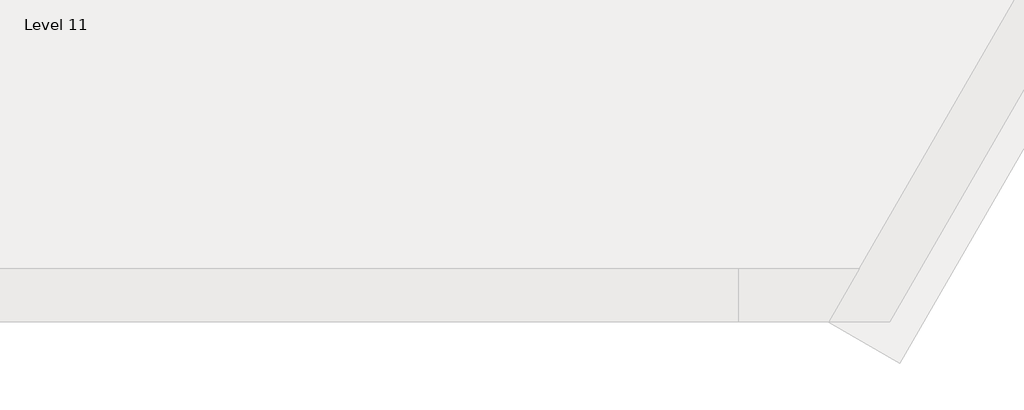
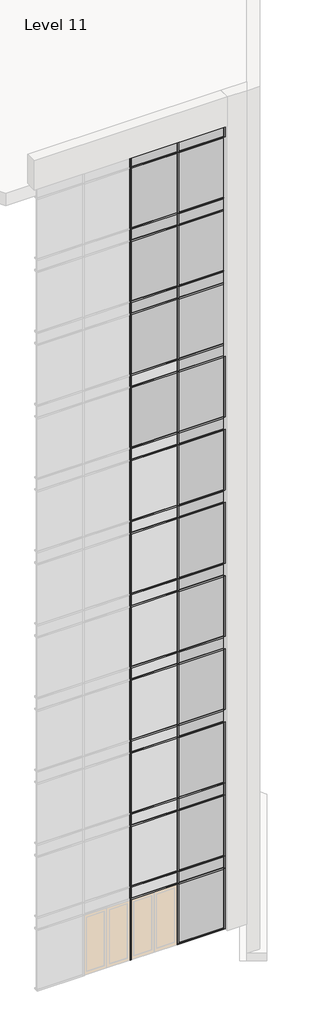
# One storey, part 3 of 6: 100 members, 29 plates.
"""IFC4 building model written with IfcOpenShell, lengths in millimetres."""

import ifcopenshell
import ifcopenshell.guid

model = None  # the IFC model being written
_history = None  # IfcOwnerHistory: only IFC2X3 demands one
_inside = {}  # id of a spatial element -> (the spatial element, [elements in it])
_under = {}  # id of a project, library or spatial element -> (it, [spatial elements below it])
_declared = {}  # id of a project -> (the project, [libraries it declares])
_typed = {}  # id of a type object -> (the type object, [elements of that type])
_made_of = {}  # id of a material, layer set ... -> (it, [elements and type objects made of it])


def new_model(schema):
    """Start an empty IFC model of exactly this schema.

    Asked for "IFC4X3", IfcOpenShell would pick the latest addendum, in which some entities
    have other attributes; the version numbers below select the first issue.
    IFC2X3 requires an IfcOwnerHistory on every rooted entity: one is made here for all.
    """
    global model, _history
    if schema == "IFC4X3":
        model = ifcopenshell.file(schema_version=(4, 3, 0, 0))
    else:
        model = ifcopenshell.file(schema=schema)
    _inside.clear()
    _under.clear()
    _declared.clear()
    _typed.clear()
    _made_of.clear()
    _history = None
    if model.schema == "IFC2X3":
        org = make("IfcOrganization", Name="unknown")
        user = make(
            "IfcPersonAndOrganization",
            ThePerson=make("IfcPerson", FamilyName="unknown"),
            TheOrganization=org,
        )
        app = make(
            "IfcApplication",
            ApplicationDeveloper=org,
            Version="unknown",
            ApplicationFullName="unknown",
            ApplicationIdentifier="unknown",
        )
        _history = make(
            "IfcOwnerHistory",
            OwningUser=user,
            OwningApplication=app,
            ChangeAction="ADDED",
            CreationDate=0,
        )
    return model


def make(cls, **values):
    """One entity of the class cls with the attributes given. An attribute that is None is left unset."""
    return model.create_entity(
        cls, **{name: value for name, value in values.items() if value is not None}
    )


def rooted(cls, **values):
    """An entity with a GlobalId (a new one), such as an element, a storey or a relation."""
    return make(cls, GlobalId=ifcopenshell.guid.new(), OwnerHistory=_history, **values)


def si_unit(unit_type, name, prefix=None):
    """IfcSIUnit, for example si_unit("LENGTHUNIT", "METRE", prefix="MILLI")."""
    return make("IfcSIUnit", UnitType=unit_type, Prefix=prefix, Name=name)


def assignment(units):
    """IfcUnitAssignment: the units of a project."""
    return None if units is None else make("IfcUnitAssignment", Units=units)


def point(xyz):
    """IfcCartesianPoint."""
    return None if xyz is None else make("IfcCartesianPoint", Coordinates=xyz)


def direction(xyz):
    """IfcDirection."""
    return None if xyz is None else make("IfcDirection", DirectionRatios=xyz)


def frame(location, z_axis=None, x_axis=None):
    """IfcAxis2Placement3D, a coordinate frame: its origin and axes. An axis left out is left unset."""
    return make(
        "IfcAxis2Placement3D",
        Location=point(location),
        Axis=direction(z_axis),
        RefDirection=direction(x_axis),
    )


def origin():
    """The frame at (0, 0, 0) with its axes left unset."""
    return frame((0.0, 0.0, 0.0))


def origin_with_axes():
    """The frame at (0, 0, 0) with the z axis (0, 0, 1) and the x axis (1, 0, 0) written out."""
    return frame((0.0, 0.0, 0.0), z_axis=(0.0, 0.0, 1.0), x_axis=(1.0, 0.0, 0.0))


def place(relative_to, where):
    """IfcLocalPlacement: puts the frame where relative to a parent placement (None: the world)."""
    return make(
        "IfcLocalPlacement", PlacementRelTo=relative_to, RelativePlacement=where
    )


def context(
    kind, dimensions, precision=None, world=None, true_north=None, identifier=None
):
    """IfcGeometricRepresentationContext, for example the 3D "Model" context."""
    return make(
        "IfcGeometricRepresentationContext",
        ContextIdentifier=identifier,
        ContextType=kind,
        CoordinateSpaceDimension=dimensions,
        Precision=precision,
        WorldCoordinateSystem=world,
        TrueNorth=true_north,
    )


def project(units=None, contexts=None):
    """IfcProject with its units and contexts."""
    return rooted(
        "IfcProject",
        Name="project",
        RepresentationContexts=contexts,
        UnitsInContext=assignment(units),
    )


def spatial(cls, under=None, at=None, **own):
    """A site, building, storey or space (cls), placed at a placement, below another one or the project."""
    s = rooted(cls, ObjectPlacement=at, **own)
    if under is not None:
        _under.setdefault(under.id(), (under, []))[1].append(s)
    return s


def polyline(points):
    """IfcPolyline through the points."""
    return make("IfcPolyline", Points=[point(p) for p in points])


def outline(outer, holes=None, kind="AREA"):
    """IfcArbitraryClosedProfileDef: a profile drawn as a closed curve; with holes, ...WithVoids."""
    if holes is None:
        return make("IfcArbitraryClosedProfileDef", ProfileType=kind, OuterCurve=outer)
    return make(
        "IfcArbitraryProfileDefWithVoids",
        ProfileType=kind,
        OuterCurve=outer,
        InnerCurves=holes,
    )


def extrude(swept, where, along, depth):
    """IfcExtrudedAreaSolid: the profile swept, set in the frame where, extruded along a direction by depth."""
    return make(
        "IfcExtrudedAreaSolid",
        SweptArea=swept,
        Position=where,
        ExtrudedDirection=direction(along),
        Depth=depth,
    )


def shape(context_of_items, identifier, shape_type, items):
    """IfcShapeRepresentation: the items that make up one representation, for example the "Body"."""
    return make(
        "IfcShapeRepresentation",
        ContextOfItems=context_of_items,
        RepresentationIdentifier=identifier,
        RepresentationType=shape_type,
        Items=items,
    )


def source(mapping_origin, context_of_items, identifier, shape_type, items):
    """IfcRepresentationMap: a shape defined once, which mapped items show again and again."""
    return make(
        "IfcRepresentationMap",
        MappingOrigin=mapping_origin,
        MappedRepresentation=shape(context_of_items, identifier, shape_type, items),
    )


def transform(
    local_origin,
    x_axis=None,
    y_axis=None,
    z_axis=None,
    scale=None,
    scale2=None,
    scale3=None,
    uniform=True,
):
    """IfcCartesianTransformationOperator3D, or its non-uniform kind. x_axis, y_axis, z_axis: its Axis1, 2, 3."""
    if uniform:
        return make(
            "IfcCartesianTransformationOperator3D",
            Axis1=direction(x_axis),
            Axis2=direction(y_axis),
            LocalOrigin=point(local_origin),
            Scale=scale,
            Axis3=direction(z_axis),
        )
    return make(
        "IfcCartesianTransformationOperator3DnonUniform",
        Axis1=direction(x_axis),
        Axis2=direction(y_axis),
        LocalOrigin=point(local_origin),
        Scale=scale,
        Axis3=direction(z_axis),
        Scale2=scale2,
        Scale3=scale3,
    )


def mapped(mapping_source, mapping_target):
    """IfcMappedItem: shows the shape of a source again, moved by a transform."""
    return make(
        "IfcMappedItem", MappingSource=mapping_source, MappingTarget=mapping_target
    )


def made_of(thing, what):
    """Note that an element or type object is made of a material, layer set ...; save() writes the relation."""
    if what is not None:
        _made_of.setdefault(what.id(), (what, []))[1].append(thing)
    return thing


def element(
    cls,
    number,
    at=None,
    inside=None,
    cuts=None,
    type_object=None,
    material=None,
    context=None,
    identifier="Body",
    shape_type=None,
    held_by="IfcProductDefinitionShape",
    body=None,
    shapes=None,
    **own,
):
    """One element of the class cls, such as IfcWall. Its Tag is "e" and its number.

    at: its placement. inside: the storey or other place that contains it. cuts: it is an
    opening in that element (IfcRelVoidsElement). A single representation is given by context,
    identifier, shape_type and body (its items); several are given by shapes. held_by: the class
    of the entity that holds the representations. save() writes the other relations.
    """
    e = rooted(cls, Tag="e%d" % number, ObjectPlacement=at, **own)
    if body is not None:
        shapes = [shape(context, identifier, shape_type, body)]
    if shapes is not None:
        e.Representation = make(held_by, Representations=shapes)
    if inside is not None:
        _inside.setdefault(inside.id(), (inside, []))[1].append(e)
    if cuts is not None:
        rooted(
            "IfcRelVoidsElement", RelatingBuildingElement=cuts, RelatedOpeningElement=e
        )
    if type_object is not None:
        _typed.setdefault(type_object.id(), (type_object, []))[1].append(e)
    return made_of(e, material)


def aggregate(whole, parts):
    """IfcRelAggregates: a whole, such as a stair, and the parts it consists of."""
    return rooted("IfcRelAggregates", RelatingObject=whole, RelatedObjects=parts)


def save(model, path):
    """Write the relations noted so far, then the file.

    IfcRelAggregates (storeys below a building ...), IfcRelContainedInSpatialStructure (elements
    in a storey), IfcRelDefinesByType, IfcRelAssociatesMaterial and IfcRelDeclares: one each for
    every whole, place, type object, material and project.
    """
    for whole, parts in _under.values():
        aggregate(whole, parts)
    for where, things in _inside.values():
        rooted(
            "IfcRelContainedInSpatialStructure",
            RelatedElements=things,
            RelatingStructure=where,
        )
    for kind, things in _typed.values():
        rooted("IfcRelDefinesByType", RelatedObjects=things, RelatingType=kind)
    for what, things in _made_of.values():
        rooted("IfcRelAssociatesMaterial", RelatedObjects=things, RelatingMaterial=what)
    for by, libraries in _declared.values():
        rooted("IfcRelDeclares", RelatingContext=by, RelatedDefinitions=libraries)
    model.write(path)


def rectangular_mullion_50x150mm_86d49a4b(model_context):
    return source(origin(), model_context, "Body", "SweptSolid", [
        extrude(outline(polyline([(0.0, 75.0), (0.0, -75.0), (-50.0, -75.0), (-50.0, 75.0), (0.0, 75.0)])), frame((0.0, 0.0, -1755.0), z_axis=(0.0, 0.0, 1.0), x_axis=(1.0, 0.0, 0.0)), (0.0, 0.0, 1.0), 1755.0),
    ])


def rectangular_mullion_50x150mm_eb9201c3(model_context):
    return source(origin(), model_context, "Body", "SweptSolid", [
        extrude(outline(polyline([(25.0, 75.0), (25.0, -75.0), (-25.0, -75.0), (-25.0, 75.0), (25.0, 75.0)])), frame((0.0, 0.0, -2500.0), z_axis=(0.0, 0.0, 1.0), x_axis=(1.0, 0.0, 0.0)), (0.0, 0.0, 1.0), 2500.0),
    ])


def rectangular_mullion_50x150mm_df7bd136(model_context):
    return source(origin(), model_context, "Body", "SweptSolid", [
        extrude(outline(polyline([(25.0, 75.0), (25.0, -75.0), (-25.0, -75.0), (-25.0, 75.0), (25.0, 75.0)])), frame((0.0, 0.0, -1755.0), z_axis=(0.0, 0.0, 1.0), x_axis=(1.0, 0.0, 0.0)), (0.0, 0.0, 1.0), 1755.0),
    ])


def rectangular_mullion_50x150mm_f5b8645b(model_context):
    return source(origin(), model_context, "Body", "SweptSolid", [
        extrude(outline(polyline([(25.0, 75.0), (25.0, -75.0), (-25.0, -75.0), (-25.0, 75.0), (25.0, 75.0)])), frame((0.0, 0.0, -1780.0), z_axis=(0.0, 0.0, 1.0), x_axis=(1.0, 0.0, 0.0)), (0.0, 0.0, 1.0), 1780.0),
    ])


def rectangular_mullion_50x150mm_ded00a16(model_context):
    return source(origin(), model_context, "Body", "SweptSolid", [
        extrude(outline(polyline([(0.0, 75.0), (0.0, -75.0), (-50.0, -75.0), (-50.0, 75.0), (0.0, 75.0)])), frame((0.0, 0.0, -1780.0), z_axis=(0.0, 0.0, 1.0), x_axis=(1.0, 0.0, 0.0)), (0.0, 0.0, 1.0), 1780.0),
    ])


def rectangular_mullion_50x150mm_22f77a7a(model_context):
    return source(origin(), model_context, "Body", "SweptSolid", [
        extrude(outline(polyline([(25.0, 75.0), (25.0, -75.0), (-25.0, -75.0), (-25.0, 75.0), (25.0, 75.0)])), frame((0.0, 0.0, -500.0), z_axis=(0.0, 0.0, 1.0), x_axis=(1.0, 0.0, 0.0)), (0.0, 0.0, 1.0), 500.0),
    ])


def rectangular_mullion_50x150mm_b3666dbd(model_context):
    return source(origin(), model_context, "Body", "SweptSolid", [
        extrude(outline(polyline([(0.0, 75.0), (0.0, -75.0), (-50.0, -75.0), (-50.0, 75.0), (0.0, 75.0)])), frame((0.0, 0.0, -500.0), z_axis=(0.0, 0.0, 1.0), x_axis=(1.0, 0.0, 0.0)), (0.0, 0.0, 1.0), 500.0),
    ])


def rectangular_mullion_50x150mm_4c3b9bdb(model_context):
    return source(origin(), model_context, "Body", "SweptSolid", [
        extrude(outline(polyline([(0.0, 75.0), (0.0, -75.0), (-50.0, -75.0), (-50.0, 75.0), (0.0, 75.0)])), frame((0.0, 0.0, -2500.0), z_axis=(0.0, 0.0, 1.0), x_axis=(1.0, 0.0, 0.0)), (0.0, 0.0, 1.0), 2500.0),
    ])


def system_panel_glazed_e1ffc32d(model_context):
    return source(origin(), model_context, "Body", "SweptSolid", [
        extrude(outline(polyline([(877.5, 24.5), (-877.5, 24.5), (-877.5, 49.5), (877.5, 49.5), (877.5, 24.5)])), origin_with_axes(), (0.0, 0.0, 1.0), 2425.0),
    ])


def system_panel_glazed_b225d226(model_context):
    return source(origin(), model_context, "Body", "SweptSolid", [
        extrude(outline(polyline([(877.5, 24.5), (-877.5, 24.5), (-877.5, 49.5), (877.5, 49.5), (877.5, 24.5)])), origin_with_axes(), (0.0, 0.0, 1.0), 450.0),
    ])


def system_panel_glazed_87c86ac8(model_context):
    return source(origin(), model_context, "Body", "SweptSolid", [
        extrude(outline(polyline([(890.0, 24.5), (-890.0, 24.5), (-890.0, 49.5), (890.0, 49.5), (890.0, 24.5)])), origin_with_axes(), (0.0, 0.0, 1.0), 450.0),
    ])


def system_panel_glazed_9668c591(model_context):
    return source(origin(), model_context, "Body", "SweptSolid", [
        extrude(outline(polyline([(877.5, 24.5), (-877.5, 24.5), (-877.5, 49.5), (877.5, 49.5), (877.5, 24.5)])), origin_with_axes(), (0.0, 0.0, 1.0), 2450.0),
    ])


def system_panel_glazed_3dade0f0(model_context):
    return source(origin(), model_context, "Body", "SweptSolid", [
        extrude(outline(polyline([(890.0, 24.5), (-890.0, 24.5), (-890.0, 49.5), (890.0, 49.5), (890.0, 24.5)])), origin_with_axes(), (0.0, 0.0, 1.0), 2450.0),
    ])


def system_panel_glazed_44ebf714(model_context):
    return source(origin(), model_context, "Body", "SweptSolid", [
        extrude(outline(polyline([(877.5, 24.5), (-877.5, 24.5), (-877.5, 49.5), (877.5, 49.5), (877.5, 24.5)])), origin_with_axes(), (0.0, 0.0, 1.0), 425.0),
    ])


def system_panel_glazed_68b51738(model_context):
    return source(origin(), model_context, "Body", "SweptSolid", [
        extrude(outline(polyline([(890.0, 24.5), (-890.0, 24.5), (-890.0, 49.5), (890.0, 49.5), (890.0, 24.5)])), origin_with_axes(), (0.0, 0.0, 1.0), 425.0),
    ])


model = new_model("IFC4")

# Units and contexts
model_context = context("Model", 3, world=origin())
ifc_project = project(units=[si_unit("LENGTHUNIT", "METRE", prefix="MILLI")], contexts=[model_context])

# Site, building, storey
site = spatial("IfcSite", under=ifc_project)
building = spatial("IfcBuilding", under=site)
storey = spatial("IfcBuildingStorey", under=building, Name="Level 11", Elevation=33000.0)

# Members
placement = place(None, origin())
rectangular_mullion_50x150mm_shape = rectangular_mullion_50x150mm_86d49a4b(model_context)
element("IfcMember", 1, ObjectType="Rectangular Mullion : 50x150mm", at=placement, inside=storey, context=model_context, shape_type="MappedRepresentation", body=[
    mapped(rectangular_mullion_50x150mm_shape, transform((3638.5639559, -8316.0631989, 0.0), x_axis=(0.0, 0.0, -1.0), y_axis=(0.0, 1.0, 0.0), z_axis=(1.0, 0.0, 0.0))),
])
rectangular_mullion_50x150mm_2_shape = rectangular_mullion_50x150mm_eb9201c3(model_context)
element("IfcMember", 2, ObjectType="Rectangular Mullion : 50x150mm", at=placement, inside=storey, context=model_context, shape_type="MappedRepresentation", body=[
    mapped(rectangular_mullion_50x150mm_2_shape, transform((1858.5639559, -8316.0631989, 0.0), x_axis=(-1.0, 0.0, 0.0), y_axis=(0.0, 1.0, 0.0), z_axis=(0.0, 0.0, -1.0))),
])
element("IfcMember", 3, ObjectType="Rectangular Mullion : 50x150mm", at=placement, inside=storey, context=model_context, shape_type="MappedRepresentation", body=[
    mapped(rectangular_mullion_50x150mm_2_shape, transform((28.5639559, -8316.0631989, 0.0), x_axis=(-1.0, 0.0, 0.0), y_axis=(0.0, 1.0, 0.0), z_axis=(0.0, 0.0, -1.0))),
])
rectangular_mullion_50x150mm_3_shape = rectangular_mullion_50x150mm_df7bd136(model_context)
element("IfcMember", 4, ObjectType="Rectangular Mullion : 50x150mm", at=placement, inside=storey, context=model_context, shape_type="MappedRepresentation", body=[
    mapped(rectangular_mullion_50x150mm_3_shape, transform((1883.5639559, -8316.0631989, 2500.0), x_axis=(0.0, 0.0, 1.0), y_axis=(0.0, 1.0, 0.0), z_axis=(-1.0, 0.0, 0.0))),
])
element("IfcMember", 5, ObjectType="Rectangular Mullion : 50x150mm", at=placement, inside=storey, context=model_context, shape_type="MappedRepresentation", body=[
    mapped(rectangular_mullion_50x150mm_3_shape, transform((1883.5639559, -8316.0631989, 5500.0), x_axis=(0.0, 0.0, 1.0), y_axis=(0.0, 1.0, 0.0), z_axis=(-1.0, 0.0, 0.0))),
])
element("IfcMember", 6, ObjectType="Rectangular Mullion : 50x150mm", at=placement, inside=storey, context=model_context, shape_type="MappedRepresentation", body=[
    mapped(rectangular_mullion_50x150mm_3_shape, transform((1883.5639559, -8316.0631989, 8500.0), x_axis=(0.0, 0.0, 1.0), y_axis=(0.0, 1.0, 0.0), z_axis=(-1.0, 0.0, 0.0))),
])
element("IfcMember", 7, ObjectType="Rectangular Mullion : 50x150mm", at=placement, inside=storey, context=model_context, shape_type="MappedRepresentation", body=[
    mapped(rectangular_mullion_50x150mm_3_shape, transform((1883.5639559, -8316.0631989, 11500.0), x_axis=(0.0, 0.0, 1.0), y_axis=(0.0, 1.0, 0.0), z_axis=(-1.0, 0.0, 0.0))),
])
element("IfcMember", 8, ObjectType="Rectangular Mullion : 50x150mm", at=placement, inside=storey, context=model_context, shape_type="MappedRepresentation", body=[
    mapped(rectangular_mullion_50x150mm_3_shape, transform((1883.5639559, -8316.0631989, 14500.0), x_axis=(0.0, 0.0, 1.0), y_axis=(0.0, 1.0, 0.0), z_axis=(-1.0, 0.0, 0.0))),
])
element("IfcMember", 9, ObjectType="Rectangular Mullion : 50x150mm", at=placement, inside=storey, context=model_context, shape_type="MappedRepresentation", body=[
    mapped(rectangular_mullion_50x150mm_3_shape, transform((1883.5639559, -8316.0631989, 17500.0), x_axis=(0.0, 0.0, 1.0), y_axis=(0.0, 1.0, 0.0), z_axis=(-1.0, 0.0, 0.0))),
])
element("IfcMember", 10, ObjectType="Rectangular Mullion : 50x150mm", at=placement, inside=storey, context=model_context, shape_type="MappedRepresentation", body=[
    mapped(rectangular_mullion_50x150mm_3_shape, transform((1883.5639559, -8316.0631989, 20500.0), x_axis=(0.0, 0.0, 1.0), y_axis=(0.0, 1.0, 0.0), z_axis=(-1.0, 0.0, 0.0))),
])
element("IfcMember", 11, ObjectType="Rectangular Mullion : 50x150mm", at=placement, inside=storey, context=model_context, shape_type="MappedRepresentation", body=[
    mapped(rectangular_mullion_50x150mm_3_shape, transform((1883.5639559, -8316.0631989, 23500.0), x_axis=(0.0, 0.0, 1.0), y_axis=(0.0, 1.0, 0.0), z_axis=(-1.0, 0.0, 0.0))),
])
element("IfcMember", 12, ObjectType="Rectangular Mullion : 50x150mm", at=placement, inside=storey, context=model_context, shape_type="MappedRepresentation", body=[
    mapped(rectangular_mullion_50x150mm_3_shape, transform((1883.5639559, -8316.0631989, 3000.0), x_axis=(0.0, 0.0, 1.0), y_axis=(0.0, 1.0, 0.0), z_axis=(-1.0, 0.0, 0.0))),
])
element("IfcMember", 13, ObjectType="Rectangular Mullion : 50x150mm", at=placement, inside=storey, context=model_context, shape_type="MappedRepresentation", body=[
    mapped(rectangular_mullion_50x150mm_3_shape, transform((1883.5639559, -8316.0631989, 6000.0), x_axis=(0.0, 0.0, 1.0), y_axis=(0.0, 1.0, 0.0), z_axis=(-1.0, 0.0, 0.0))),
])
element("IfcMember", 14, ObjectType="Rectangular Mullion : 50x150mm", at=placement, inside=storey, context=model_context, shape_type="MappedRepresentation", body=[
    mapped(rectangular_mullion_50x150mm_3_shape, transform((1883.5639559, -8316.0631989, 9000.0), x_axis=(0.0, 0.0, 1.0), y_axis=(0.0, 1.0, 0.0), z_axis=(-1.0, 0.0, 0.0))),
])
element("IfcMember", 15, ObjectType="Rectangular Mullion : 50x150mm", at=placement, inside=storey, context=model_context, shape_type="MappedRepresentation", body=[
    mapped(rectangular_mullion_50x150mm_3_shape, transform((1883.5639559, -8316.0631989, 12000.0), x_axis=(0.0, 0.0, 1.0), y_axis=(0.0, 1.0, 0.0), z_axis=(-1.0, 0.0, 0.0))),
])
element("IfcMember", 16, ObjectType="Rectangular Mullion : 50x150mm", at=placement, inside=storey, context=model_context, shape_type="MappedRepresentation", body=[
    mapped(rectangular_mullion_50x150mm_3_shape, transform((1883.5639559, -8316.0631989, 15000.0), x_axis=(0.0, 0.0, 1.0), y_axis=(0.0, 1.0, 0.0), z_axis=(-1.0, 0.0, 0.0))),
])
element("IfcMember", 17, ObjectType="Rectangular Mullion : 50x150mm", at=placement, inside=storey, context=model_context, shape_type="MappedRepresentation", body=[
    mapped(rectangular_mullion_50x150mm_3_shape, transform((1883.5639559, -8316.0631989, 18000.0), x_axis=(0.0, 0.0, 1.0), y_axis=(0.0, 1.0, 0.0), z_axis=(-1.0, 0.0, 0.0))),
])
element("IfcMember", 18, ObjectType="Rectangular Mullion : 50x150mm", at=placement, inside=storey, context=model_context, shape_type="MappedRepresentation", body=[
    mapped(rectangular_mullion_50x150mm_3_shape, transform((1883.5639559, -8316.0631989, 21000.0), x_axis=(0.0, 0.0, 1.0), y_axis=(0.0, 1.0, 0.0), z_axis=(-1.0, 0.0, 0.0))),
])
element("IfcMember", 19, ObjectType="Rectangular Mullion : 50x150mm", at=placement, inside=storey, context=model_context, shape_type="MappedRepresentation", body=[
    mapped(rectangular_mullion_50x150mm_3_shape, transform((1883.5639559, -8316.0631989, 24000.0), x_axis=(0.0, 0.0, 1.0), y_axis=(0.0, 1.0, 0.0), z_axis=(-1.0, 0.0, 0.0))),
])
element("IfcMember", 20, ObjectType="Rectangular Mullion : 50x150mm", at=placement, inside=storey, context=model_context, shape_type="MappedRepresentation", body=[
    mapped(rectangular_mullion_50x150mm_3_shape, transform((1883.5639559, -8316.0631989, 27000.0), x_axis=(0.0, 0.0, 1.0), y_axis=(0.0, 1.0, 0.0), z_axis=(-1.0, 0.0, 0.0))),
])
element("IfcMember", 21, ObjectType="Rectangular Mullion : 50x150mm", at=placement, inside=storey, context=model_context, shape_type="MappedRepresentation", body=[
    mapped(rectangular_mullion_50x150mm_3_shape, transform((1883.5639559, -8316.0631989, 26500.0), x_axis=(0.0, 0.0, 1.0), y_axis=(0.0, 1.0, 0.0), z_axis=(-1.0, 0.0, 0.0))),
])
element("IfcMember", 22, ObjectType="Rectangular Mullion : 50x150mm", at=placement, inside=storey, context=model_context, shape_type="MappedRepresentation", body=[
    mapped(rectangular_mullion_50x150mm_3_shape, transform((1883.5639559, -8316.0631989, 30000.0), x_axis=(0.0, 0.0, 1.0), y_axis=(0.0, 1.0, 0.0), z_axis=(-1.0, 0.0, 0.0))),
])
element("IfcMember", 23, ObjectType="Rectangular Mullion : 50x150mm", at=placement, inside=storey, context=model_context, shape_type="MappedRepresentation", body=[
    mapped(rectangular_mullion_50x150mm_3_shape, transform((1883.5639559, -8316.0631989, 29500.0), x_axis=(0.0, 0.0, 1.0), y_axis=(0.0, 1.0, 0.0), z_axis=(-1.0, 0.0, 0.0))),
])
element("IfcMember", 24, ObjectType="Rectangular Mullion : 50x150mm", at=placement, inside=storey, context=model_context, shape_type="MappedRepresentation", body=[
    mapped(rectangular_mullion_50x150mm_3_shape, transform((1883.5639559, -8316.0631989, 32500.0), x_axis=(0.0, 0.0, 1.0), y_axis=(0.0, 1.0, 0.0), z_axis=(-1.0, 0.0, 0.0))),
])
rectangular_mullion_50x150mm_4_shape = rectangular_mullion_50x150mm_f5b8645b(model_context)
element("IfcMember", 25, ObjectType="Rectangular Mullion : 50x150mm", at=placement, inside=storey, context=model_context, shape_type="MappedRepresentation", body=[
    mapped(rectangular_mullion_50x150mm_4_shape, transform((53.5639559, -8316.0631989, 2500.0), x_axis=(0.0, 0.0, 1.0), y_axis=(0.0, 1.0, 0.0), z_axis=(-1.0, 0.0, 0.0))),
])
element("IfcMember", 26, ObjectType="Rectangular Mullion : 50x150mm", at=placement, inside=storey, context=model_context, shape_type="MappedRepresentation", body=[
    mapped(rectangular_mullion_50x150mm_4_shape, transform((53.5639559, -8316.0631989, 5500.0), x_axis=(0.0, 0.0, 1.0), y_axis=(0.0, 1.0, 0.0), z_axis=(-1.0, 0.0, 0.0))),
])
element("IfcMember", 27, ObjectType="Rectangular Mullion : 50x150mm", at=placement, inside=storey, context=model_context, shape_type="MappedRepresentation", body=[
    mapped(rectangular_mullion_50x150mm_4_shape, transform((53.5639559, -8316.0631989, 8500.0), x_axis=(0.0, 0.0, 1.0), y_axis=(0.0, 1.0, 0.0), z_axis=(-1.0, 0.0, 0.0))),
])
element("IfcMember", 28, ObjectType="Rectangular Mullion : 50x150mm", at=placement, inside=storey, context=model_context, shape_type="MappedRepresentation", body=[
    mapped(rectangular_mullion_50x150mm_4_shape, transform((53.5639559, -8316.0631989, 11500.0), x_axis=(0.0, 0.0, 1.0), y_axis=(0.0, 1.0, 0.0), z_axis=(-1.0, 0.0, 0.0))),
])
element("IfcMember", 29, ObjectType="Rectangular Mullion : 50x150mm", at=placement, inside=storey, context=model_context, shape_type="MappedRepresentation", body=[
    mapped(rectangular_mullion_50x150mm_4_shape, transform((53.5639559, -8316.0631989, 14500.0), x_axis=(0.0, 0.0, 1.0), y_axis=(0.0, 1.0, 0.0), z_axis=(-1.0, 0.0, 0.0))),
])
element("IfcMember", 30, ObjectType="Rectangular Mullion : 50x150mm", at=placement, inside=storey, context=model_context, shape_type="MappedRepresentation", body=[
    mapped(rectangular_mullion_50x150mm_4_shape, transform((53.5639559, -8316.0631989, 17500.0), x_axis=(0.0, 0.0, 1.0), y_axis=(0.0, 1.0, 0.0), z_axis=(-1.0, 0.0, 0.0))),
])
element("IfcMember", 31, ObjectType="Rectangular Mullion : 50x150mm", at=placement, inside=storey, context=model_context, shape_type="MappedRepresentation", body=[
    mapped(rectangular_mullion_50x150mm_4_shape, transform((53.5639559, -8316.0631989, 20500.0), x_axis=(0.0, 0.0, 1.0), y_axis=(0.0, 1.0, 0.0), z_axis=(-1.0, 0.0, 0.0))),
])
element("IfcMember", 32, ObjectType="Rectangular Mullion : 50x150mm", at=placement, inside=storey, context=model_context, shape_type="MappedRepresentation", body=[
    mapped(rectangular_mullion_50x150mm_4_shape, transform((53.5639559, -8316.0631989, 23500.0), x_axis=(0.0, 0.0, 1.0), y_axis=(0.0, 1.0, 0.0), z_axis=(-1.0, 0.0, 0.0))),
])
element("IfcMember", 33, ObjectType="Rectangular Mullion : 50x150mm", at=placement, inside=storey, context=model_context, shape_type="MappedRepresentation", body=[
    mapped(rectangular_mullion_50x150mm_4_shape, transform((53.5639559, -8316.0631989, 3000.0), x_axis=(0.0, 0.0, 1.0), y_axis=(0.0, 1.0, 0.0), z_axis=(-1.0, 0.0, 0.0))),
])
element("IfcMember", 34, ObjectType="Rectangular Mullion : 50x150mm", at=placement, inside=storey, context=model_context, shape_type="MappedRepresentation", body=[
    mapped(rectangular_mullion_50x150mm_4_shape, transform((53.5639559, -8316.0631989, 6000.0), x_axis=(0.0, 0.0, 1.0), y_axis=(0.0, 1.0, 0.0), z_axis=(-1.0, 0.0, 0.0))),
])
element("IfcMember", 35, ObjectType="Rectangular Mullion : 50x150mm", at=placement, inside=storey, context=model_context, shape_type="MappedRepresentation", body=[
    mapped(rectangular_mullion_50x150mm_4_shape, transform((53.5639559, -8316.0631989, 9000.0), x_axis=(0.0, 0.0, 1.0), y_axis=(0.0, 1.0, 0.0), z_axis=(-1.0, 0.0, 0.0))),
])
element("IfcMember", 36, ObjectType="Rectangular Mullion : 50x150mm", at=placement, inside=storey, context=model_context, shape_type="MappedRepresentation", body=[
    mapped(rectangular_mullion_50x150mm_4_shape, transform((53.5639559, -8316.0631989, 12000.0), x_axis=(0.0, 0.0, 1.0), y_axis=(0.0, 1.0, 0.0), z_axis=(-1.0, 0.0, 0.0))),
])
element("IfcMember", 37, ObjectType="Rectangular Mullion : 50x150mm", at=placement, inside=storey, context=model_context, shape_type="MappedRepresentation", body=[
    mapped(rectangular_mullion_50x150mm_4_shape, transform((53.5639559, -8316.0631989, 15000.0), x_axis=(0.0, 0.0, 1.0), y_axis=(0.0, 1.0, 0.0), z_axis=(-1.0, 0.0, 0.0))),
])
element("IfcMember", 38, ObjectType="Rectangular Mullion : 50x150mm", at=placement, inside=storey, context=model_context, shape_type="MappedRepresentation", body=[
    mapped(rectangular_mullion_50x150mm_4_shape, transform((53.5639559, -8316.0631989, 18000.0), x_axis=(0.0, 0.0, 1.0), y_axis=(0.0, 1.0, 0.0), z_axis=(-1.0, 0.0, 0.0))),
])
element("IfcMember", 39, ObjectType="Rectangular Mullion : 50x150mm", at=placement, inside=storey, context=model_context, shape_type="MappedRepresentation", body=[
    mapped(rectangular_mullion_50x150mm_4_shape, transform((53.5639559, -8316.0631989, 21000.0), x_axis=(0.0, 0.0, 1.0), y_axis=(0.0, 1.0, 0.0), z_axis=(-1.0, 0.0, 0.0))),
])
element("IfcMember", 40, ObjectType="Rectangular Mullion : 50x150mm", at=placement, inside=storey, context=model_context, shape_type="MappedRepresentation", body=[
    mapped(rectangular_mullion_50x150mm_4_shape, transform((53.5639559, -8316.0631989, 24000.0), x_axis=(0.0, 0.0, 1.0), y_axis=(0.0, 1.0, 0.0), z_axis=(-1.0, 0.0, 0.0))),
])
element("IfcMember", 41, ObjectType="Rectangular Mullion : 50x150mm", at=placement, inside=storey, context=model_context, shape_type="MappedRepresentation", body=[
    mapped(rectangular_mullion_50x150mm_4_shape, transform((53.5639559, -8316.0631989, 27000.0), x_axis=(0.0, 0.0, 1.0), y_axis=(0.0, 1.0, 0.0), z_axis=(-1.0, 0.0, 0.0))),
])
element("IfcMember", 42, ObjectType="Rectangular Mullion : 50x150mm", at=placement, inside=storey, context=model_context, shape_type="MappedRepresentation", body=[
    mapped(rectangular_mullion_50x150mm_4_shape, transform((53.5639559, -8316.0631989, 26500.0), x_axis=(0.0, 0.0, 1.0), y_axis=(0.0, 1.0, 0.0), z_axis=(-1.0, 0.0, 0.0))),
])
element("IfcMember", 43, ObjectType="Rectangular Mullion : 50x150mm", at=placement, inside=storey, context=model_context, shape_type="MappedRepresentation", body=[
    mapped(rectangular_mullion_50x150mm_4_shape, transform((53.5639559, -8316.0631989, 30000.0), x_axis=(0.0, 0.0, 1.0), y_axis=(0.0, 1.0, 0.0), z_axis=(-1.0, 0.0, 0.0))),
])
element("IfcMember", 44, ObjectType="Rectangular Mullion : 50x150mm", at=placement, inside=storey, context=model_context, shape_type="MappedRepresentation", body=[
    mapped(rectangular_mullion_50x150mm_4_shape, transform((53.5639559, -8316.0631989, 29500.0), x_axis=(0.0, 0.0, 1.0), y_axis=(0.0, 1.0, 0.0), z_axis=(-1.0, 0.0, 0.0))),
])
element("IfcMember", 45, ObjectType="Rectangular Mullion : 50x150mm", at=placement, inside=storey, context=model_context, shape_type="MappedRepresentation", body=[
    mapped(rectangular_mullion_50x150mm_4_shape, transform((53.5639559, -8316.0631989, 32500.0), x_axis=(0.0, 0.0, 1.0), y_axis=(0.0, 1.0, 0.0), z_axis=(-1.0, 0.0, 0.0))),
])
element("IfcMember", 46, ObjectType="Rectangular Mullion : 50x150mm", at=placement, inside=storey, context=model_context, shape_type="MappedRepresentation", body=[
    mapped(rectangular_mullion_50x150mm_shape, transform((1883.5639559, -8316.0631989, 33000.0), x_axis=(0.0, 0.0, 1.0), y_axis=(0.0, 1.0, 0.0), z_axis=(-1.0, 0.0, 0.0))),
])
rectangular_mullion_50x150mm_5_shape = rectangular_mullion_50x150mm_ded00a16(model_context)
element("IfcMember", 47, ObjectType="Rectangular Mullion : 50x150mm", at=placement, inside=storey, context=model_context, shape_type="MappedRepresentation", body=[
    mapped(rectangular_mullion_50x150mm_5_shape, transform((53.5639559, -8316.0631989, 33000.0), x_axis=(0.0, 0.0, 1.0), y_axis=(0.0, 1.0, 0.0), z_axis=(-1.0, 0.0, 0.0))),
])
rectangular_mullion_50x150mm_6_shape = rectangular_mullion_50x150mm_22f77a7a(model_context)
element("IfcMember", 48, ObjectType="Rectangular Mullion : 50x150mm", at=placement, inside=storey, context=model_context, shape_type="MappedRepresentation", body=[
    mapped(rectangular_mullion_50x150mm_6_shape, transform((1858.5639559, -8316.0631989, 2500.0), x_axis=(-1.0, 0.0, 0.0), y_axis=(0.0, 1.0, 0.0), z_axis=(0.0, 0.0, -1.0))),
])
element("IfcMember", 49, ObjectType="Rectangular Mullion : 50x150mm", at=placement, inside=storey, context=model_context, shape_type="MappedRepresentation", body=[
    mapped(rectangular_mullion_50x150mm_6_shape, transform((1858.5639559, -8316.0631989, 5500.0), x_axis=(-1.0, 0.0, 0.0), y_axis=(0.0, 1.0, 0.0), z_axis=(0.0, 0.0, -1.0))),
])
element("IfcMember", 50, ObjectType="Rectangular Mullion : 50x150mm", at=placement, inside=storey, context=model_context, shape_type="MappedRepresentation", body=[
    mapped(rectangular_mullion_50x150mm_6_shape, transform((1858.5639559, -8316.0631989, 8500.0), x_axis=(-1.0, 0.0, 0.0), y_axis=(0.0, 1.0, 0.0), z_axis=(0.0, 0.0, -1.0))),
])
element("IfcMember", 51, ObjectType="Rectangular Mullion : 50x150mm", at=placement, inside=storey, context=model_context, shape_type="MappedRepresentation", body=[
    mapped(rectangular_mullion_50x150mm_6_shape, transform((1858.5639559, -8316.0631989, 11500.0), x_axis=(-1.0, 0.0, 0.0), y_axis=(0.0, 1.0, 0.0), z_axis=(0.0, 0.0, -1.0))),
])
element("IfcMember", 52, ObjectType="Rectangular Mullion : 50x150mm", at=placement, inside=storey, context=model_context, shape_type="MappedRepresentation", body=[
    mapped(rectangular_mullion_50x150mm_6_shape, transform((1858.5639559, -8316.0631989, 14500.0), x_axis=(-1.0, 0.0, 0.0), y_axis=(0.0, 1.0, 0.0), z_axis=(0.0, 0.0, -1.0))),
])
element("IfcMember", 53, ObjectType="Rectangular Mullion : 50x150mm", at=placement, inside=storey, context=model_context, shape_type="MappedRepresentation", body=[
    mapped(rectangular_mullion_50x150mm_6_shape, transform((1858.5639559, -8316.0631989, 17500.0), x_axis=(-1.0, 0.0, 0.0), y_axis=(0.0, 1.0, 0.0), z_axis=(0.0, 0.0, -1.0))),
])
element("IfcMember", 54, ObjectType="Rectangular Mullion : 50x150mm", at=placement, inside=storey, context=model_context, shape_type="MappedRepresentation", body=[
    mapped(rectangular_mullion_50x150mm_6_shape, transform((1858.5639559, -8316.0631989, 20500.0), x_axis=(-1.0, 0.0, 0.0), y_axis=(0.0, 1.0, 0.0), z_axis=(0.0, 0.0, -1.0))),
])
element("IfcMember", 55, ObjectType="Rectangular Mullion : 50x150mm", at=placement, inside=storey, context=model_context, shape_type="MappedRepresentation", body=[
    mapped(rectangular_mullion_50x150mm_6_shape, transform((1858.5639559, -8316.0631989, 23500.0), x_axis=(-1.0, 0.0, 0.0), y_axis=(0.0, 1.0, 0.0), z_axis=(0.0, 0.0, -1.0))),
])
element("IfcMember", 56, ObjectType="Rectangular Mullion : 50x150mm", at=placement, inside=storey, context=model_context, shape_type="MappedRepresentation", body=[
    mapped(rectangular_mullion_50x150mm_6_shape, transform((1858.5639559, -8316.0631989, 26500.0), x_axis=(-1.0, 0.0, 0.0), y_axis=(0.0, 1.0, 0.0), z_axis=(0.0, 0.0, -1.0))),
])
element("IfcMember", 57, ObjectType="Rectangular Mullion : 50x150mm", at=placement, inside=storey, context=model_context, shape_type="MappedRepresentation", body=[
    mapped(rectangular_mullion_50x150mm_6_shape, transform((1858.5639559, -8316.0631989, 29500.0), x_axis=(-1.0, 0.0, 0.0), y_axis=(0.0, 1.0, 0.0), z_axis=(0.0, 0.0, -1.0))),
])
element("IfcMember", 58, ObjectType="Rectangular Mullion : 50x150mm", at=placement, inside=storey, context=model_context, shape_type="MappedRepresentation", body=[
    mapped(rectangular_mullion_50x150mm_6_shape, transform((28.5639559, -8316.0631989, 2500.0), x_axis=(-1.0, 0.0, 0.0), y_axis=(0.0, 1.0, 0.0), z_axis=(0.0, 0.0, -1.0))),
])
element("IfcMember", 59, ObjectType="Rectangular Mullion : 50x150mm", at=placement, inside=storey, context=model_context, shape_type="MappedRepresentation", body=[
    mapped(rectangular_mullion_50x150mm_6_shape, transform((28.5639559, -8316.0631989, 5500.0), x_axis=(-1.0, 0.0, 0.0), y_axis=(0.0, 1.0, 0.0), z_axis=(0.0, 0.0, -1.0))),
])
element("IfcMember", 60, ObjectType="Rectangular Mullion : 50x150mm", at=placement, inside=storey, context=model_context, shape_type="MappedRepresentation", body=[
    mapped(rectangular_mullion_50x150mm_6_shape, transform((28.5639559, -8316.0631989, 8500.0), x_axis=(-1.0, 0.0, 0.0), y_axis=(0.0, 1.0, 0.0), z_axis=(0.0, 0.0, -1.0))),
])
element("IfcMember", 61, ObjectType="Rectangular Mullion : 50x150mm", at=placement, inside=storey, context=model_context, shape_type="MappedRepresentation", body=[
    mapped(rectangular_mullion_50x150mm_6_shape, transform((28.5639559, -8316.0631989, 11500.0), x_axis=(-1.0, 0.0, 0.0), y_axis=(0.0, 1.0, 0.0), z_axis=(0.0, 0.0, -1.0))),
])
element("IfcMember", 62, ObjectType="Rectangular Mullion : 50x150mm", at=placement, inside=storey, context=model_context, shape_type="MappedRepresentation", body=[
    mapped(rectangular_mullion_50x150mm_6_shape, transform((28.5639559, -8316.0631989, 14500.0), x_axis=(-1.0, 0.0, 0.0), y_axis=(0.0, 1.0, 0.0), z_axis=(0.0, 0.0, -1.0))),
])
element("IfcMember", 63, ObjectType="Rectangular Mullion : 50x150mm", at=placement, inside=storey, context=model_context, shape_type="MappedRepresentation", body=[
    mapped(rectangular_mullion_50x150mm_6_shape, transform((28.5639559, -8316.0631989, 17500.0), x_axis=(-1.0, 0.0, 0.0), y_axis=(0.0, 1.0, 0.0), z_axis=(0.0, 0.0, -1.0))),
])
element("IfcMember", 64, ObjectType="Rectangular Mullion : 50x150mm", at=placement, inside=storey, context=model_context, shape_type="MappedRepresentation", body=[
    mapped(rectangular_mullion_50x150mm_6_shape, transform((28.5639559, -8316.0631989, 20500.0), x_axis=(-1.0, 0.0, 0.0), y_axis=(0.0, 1.0, 0.0), z_axis=(0.0, 0.0, -1.0))),
])
element("IfcMember", 65, ObjectType="Rectangular Mullion : 50x150mm", at=placement, inside=storey, context=model_context, shape_type="MappedRepresentation", body=[
    mapped(rectangular_mullion_50x150mm_6_shape, transform((28.5639559, -8316.0631989, 23500.0), x_axis=(-1.0, 0.0, 0.0), y_axis=(0.0, 1.0, 0.0), z_axis=(0.0, 0.0, -1.0))),
])
element("IfcMember", 66, ObjectType="Rectangular Mullion : 50x150mm", at=placement, inside=storey, context=model_context, shape_type="MappedRepresentation", body=[
    mapped(rectangular_mullion_50x150mm_6_shape, transform((28.5639559, -8316.0631989, 26500.0), x_axis=(-1.0, 0.0, 0.0), y_axis=(0.0, 1.0, 0.0), z_axis=(0.0, 0.0, -1.0))),
])
element("IfcMember", 67, ObjectType="Rectangular Mullion : 50x150mm", at=placement, inside=storey, context=model_context, shape_type="MappedRepresentation", body=[
    mapped(rectangular_mullion_50x150mm_6_shape, transform((28.5639559, -8316.0631989, 29500.0), x_axis=(-1.0, 0.0, 0.0), y_axis=(0.0, 1.0, 0.0), z_axis=(0.0, 0.0, -1.0))),
])
element("IfcMember", 68, ObjectType="Rectangular Mullion : 50x150mm", at=placement, inside=storey, context=model_context, shape_type="MappedRepresentation", body=[
    mapped(rectangular_mullion_50x150mm_2_shape, transform((1858.5639559, -8316.0631989, 3000.0), x_axis=(-1.0, 0.0, 0.0), y_axis=(0.0, 1.0, 0.0), z_axis=(0.0, 0.0, -1.0))),
])
element("IfcMember", 69, ObjectType="Rectangular Mullion : 50x150mm", at=placement, inside=storey, context=model_context, shape_type="MappedRepresentation", body=[
    mapped(rectangular_mullion_50x150mm_2_shape, transform((1858.5639559, -8316.0631989, 6000.0), x_axis=(-1.0, 0.0, 0.0), y_axis=(0.0, 1.0, 0.0), z_axis=(0.0, 0.0, -1.0))),
])
element("IfcMember", 70, ObjectType="Rectangular Mullion : 50x150mm", at=placement, inside=storey, context=model_context, shape_type="MappedRepresentation", body=[
    mapped(rectangular_mullion_50x150mm_2_shape, transform((1858.5639559, -8316.0631989, 9000.0), x_axis=(-1.0, 0.0, 0.0), y_axis=(0.0, 1.0, 0.0), z_axis=(0.0, 0.0, -1.0))),
])
element("IfcMember", 71, ObjectType="Rectangular Mullion : 50x150mm", at=placement, inside=storey, context=model_context, shape_type="MappedRepresentation", body=[
    mapped(rectangular_mullion_50x150mm_2_shape, transform((1858.5639559, -8316.0631989, 12000.0), x_axis=(-1.0, 0.0, 0.0), y_axis=(0.0, 1.0, 0.0), z_axis=(0.0, 0.0, -1.0))),
])
element("IfcMember", 72, ObjectType="Rectangular Mullion : 50x150mm", at=placement, inside=storey, context=model_context, shape_type="MappedRepresentation", body=[
    mapped(rectangular_mullion_50x150mm_2_shape, transform((1858.5639559, -8316.0631989, 15000.0), x_axis=(-1.0, 0.0, 0.0), y_axis=(0.0, 1.0, 0.0), z_axis=(0.0, 0.0, -1.0))),
])
element("IfcMember", 73, ObjectType="Rectangular Mullion : 50x150mm", at=placement, inside=storey, context=model_context, shape_type="MappedRepresentation", body=[
    mapped(rectangular_mullion_50x150mm_2_shape, transform((1858.5639559, -8316.0631989, 18000.0), x_axis=(-1.0, 0.0, 0.0), y_axis=(0.0, 1.0, 0.0), z_axis=(0.0, 0.0, -1.0))),
])
element("IfcMember", 74, ObjectType="Rectangular Mullion : 50x150mm", at=placement, inside=storey, context=model_context, shape_type="MappedRepresentation", body=[
    mapped(rectangular_mullion_50x150mm_2_shape, transform((1858.5639559, -8316.0631989, 21000.0), x_axis=(-1.0, 0.0, 0.0), y_axis=(0.0, 1.0, 0.0), z_axis=(0.0, 0.0, -1.0))),
])
element("IfcMember", 75, ObjectType="Rectangular Mullion : 50x150mm", at=placement, inside=storey, context=model_context, shape_type="MappedRepresentation", body=[
    mapped(rectangular_mullion_50x150mm_2_shape, transform((1858.5639559, -8316.0631989, 24000.0), x_axis=(-1.0, 0.0, 0.0), y_axis=(0.0, 1.0, 0.0), z_axis=(0.0, 0.0, -1.0))),
])
element("IfcMember", 76, ObjectType="Rectangular Mullion : 50x150mm", at=placement, inside=storey, context=model_context, shape_type="MappedRepresentation", body=[
    mapped(rectangular_mullion_50x150mm_2_shape, transform((1858.5639559, -8316.0631989, 27000.0), x_axis=(-1.0, 0.0, 0.0), y_axis=(0.0, 1.0, 0.0), z_axis=(0.0, 0.0, -1.0))),
])
element("IfcMember", 77, ObjectType="Rectangular Mullion : 50x150mm", at=placement, inside=storey, context=model_context, shape_type="MappedRepresentation", body=[
    mapped(rectangular_mullion_50x150mm_2_shape, transform((1858.5639559, -8316.0631989, 30000.0), x_axis=(-1.0, 0.0, 0.0), y_axis=(0.0, 1.0, 0.0), z_axis=(0.0, 0.0, -1.0))),
])
element("IfcMember", 78, ObjectType="Rectangular Mullion : 50x150mm", at=placement, inside=storey, context=model_context, shape_type="MappedRepresentation", body=[
    mapped(rectangular_mullion_50x150mm_2_shape, transform((28.5639559, -8316.0631989, 3000.0), x_axis=(-1.0, 0.0, 0.0), y_axis=(0.0, 1.0, 0.0), z_axis=(0.0, 0.0, -1.0))),
])
element("IfcMember", 79, ObjectType="Rectangular Mullion : 50x150mm", at=placement, inside=storey, context=model_context, shape_type="MappedRepresentation", body=[
    mapped(rectangular_mullion_50x150mm_2_shape, transform((28.5639559, -8316.0631989, 6000.0), x_axis=(-1.0, 0.0, 0.0), y_axis=(0.0, 1.0, 0.0), z_axis=(0.0, 0.0, -1.0))),
])
element("IfcMember", 80, ObjectType="Rectangular Mullion : 50x150mm", at=placement, inside=storey, context=model_context, shape_type="MappedRepresentation", body=[
    mapped(rectangular_mullion_50x150mm_2_shape, transform((28.5639559, -8316.0631989, 9000.0), x_axis=(-1.0, 0.0, 0.0), y_axis=(0.0, 1.0, 0.0), z_axis=(0.0, 0.0, -1.0))),
])
element("IfcMember", 81, ObjectType="Rectangular Mullion : 50x150mm", at=placement, inside=storey, context=model_context, shape_type="MappedRepresentation", body=[
    mapped(rectangular_mullion_50x150mm_2_shape, transform((28.5639559, -8316.0631989, 12000.0), x_axis=(-1.0, 0.0, 0.0), y_axis=(0.0, 1.0, 0.0), z_axis=(0.0, 0.0, -1.0))),
])
element("IfcMember", 82, ObjectType="Rectangular Mullion : 50x150mm", at=placement, inside=storey, context=model_context, shape_type="MappedRepresentation", body=[
    mapped(rectangular_mullion_50x150mm_2_shape, transform((28.5639559, -8316.0631989, 15000.0), x_axis=(-1.0, 0.0, 0.0), y_axis=(0.0, 1.0, 0.0), z_axis=(0.0, 0.0, -1.0))),
])
element("IfcMember", 83, ObjectType="Rectangular Mullion : 50x150mm", at=placement, inside=storey, context=model_context, shape_type="MappedRepresentation", body=[
    mapped(rectangular_mullion_50x150mm_2_shape, transform((28.5639559, -8316.0631989, 18000.0), x_axis=(-1.0, 0.0, 0.0), y_axis=(0.0, 1.0, 0.0), z_axis=(0.0, 0.0, -1.0))),
])
element("IfcMember", 84, ObjectType="Rectangular Mullion : 50x150mm", at=placement, inside=storey, context=model_context, shape_type="MappedRepresentation", body=[
    mapped(rectangular_mullion_50x150mm_2_shape, transform((28.5639559, -8316.0631989, 21000.0), x_axis=(-1.0, 0.0, 0.0), y_axis=(0.0, 1.0, 0.0), z_axis=(0.0, 0.0, -1.0))),
])
element("IfcMember", 85, ObjectType="Rectangular Mullion : 50x150mm", at=placement, inside=storey, context=model_context, shape_type="MappedRepresentation", body=[
    mapped(rectangular_mullion_50x150mm_2_shape, transform((28.5639559, -8316.0631989, 24000.0), x_axis=(-1.0, 0.0, 0.0), y_axis=(0.0, 1.0, 0.0), z_axis=(0.0, 0.0, -1.0))),
])
element("IfcMember", 86, ObjectType="Rectangular Mullion : 50x150mm", at=placement, inside=storey, context=model_context, shape_type="MappedRepresentation", body=[
    mapped(rectangular_mullion_50x150mm_2_shape, transform((28.5639559, -8316.0631989, 27000.0), x_axis=(-1.0, 0.0, 0.0), y_axis=(0.0, 1.0, 0.0), z_axis=(0.0, 0.0, -1.0))),
])
element("IfcMember", 87, ObjectType="Rectangular Mullion : 50x150mm", at=placement, inside=storey, context=model_context, shape_type="MappedRepresentation", body=[
    mapped(rectangular_mullion_50x150mm_2_shape, transform((28.5639559, -8316.0631989, 30000.0), x_axis=(-1.0, 0.0, 0.0), y_axis=(0.0, 1.0, 0.0), z_axis=(0.0, 0.0, -1.0))),
])
element("IfcMember", 88, ObjectType="Rectangular Mullion : 50x150mm", at=placement, inside=storey, context=model_context, shape_type="MappedRepresentation", body=[
    mapped(rectangular_mullion_50x150mm_6_shape, transform((1858.5639559, -8316.0631989, 32500.0), x_axis=(-1.0, 0.0, 0.0), y_axis=(0.0, 1.0, 0.0), z_axis=(0.0, 0.0, -1.0))),
])
element("IfcMember", 89, ObjectType="Rectangular Mullion : 50x150mm", at=placement, inside=storey, context=model_context, shape_type="MappedRepresentation", body=[
    mapped(rectangular_mullion_50x150mm_6_shape, transform((28.5639559, -8316.0631989, 32500.0), x_axis=(-1.0, 0.0, 0.0), y_axis=(0.0, 1.0, 0.0), z_axis=(0.0, 0.0, -1.0))),
])
rectangular_mullion_50x150mm_7_shape = rectangular_mullion_50x150mm_b3666dbd(model_context)
element("IfcMember", 90, ObjectType="Rectangular Mullion : 50x150mm", at=placement, inside=storey, context=model_context, shape_type="MappedRepresentation", body=[
    mapped(rectangular_mullion_50x150mm_7_shape, transform((3688.5639559, -8316.0631989, 33000.0), x_axis=(1.0, 0.0, 0.0), y_axis=(0.0, 1.0, 0.0), z_axis=(0.0, 0.0, 1.0))),
])
rectangular_mullion_50x150mm_8_shape = rectangular_mullion_50x150mm_4c3b9bdb(model_context)
element("IfcMember", 91, ObjectType="Rectangular Mullion : 50x150mm", at=placement, inside=storey, context=model_context, shape_type="MappedRepresentation", body=[
    mapped(rectangular_mullion_50x150mm_8_shape, transform((3688.5639559, -8316.0631989, 2500.0), x_axis=(1.0, 0.0, 0.0), y_axis=(0.0, 1.0, 0.0), z_axis=(0.0, 0.0, 1.0))),
])
element("IfcMember", 92, ObjectType="Rectangular Mullion : 50x150mm", at=placement, inside=storey, context=model_context, shape_type="MappedRepresentation", body=[
    mapped(rectangular_mullion_50x150mm_8_shape, transform((3688.5639559, -8316.0631989, 5500.0), x_axis=(1.0, 0.0, 0.0), y_axis=(0.0, 1.0, 0.0), z_axis=(0.0, 0.0, 1.0))),
])
element("IfcMember", 93, ObjectType="Rectangular Mullion : 50x150mm", at=placement, inside=storey, context=model_context, shape_type="MappedRepresentation", body=[
    mapped(rectangular_mullion_50x150mm_8_shape, transform((3688.5639559, -8316.0631989, 8500.0), x_axis=(1.0, 0.0, 0.0), y_axis=(0.0, 1.0, 0.0), z_axis=(0.0, 0.0, 1.0))),
])
element("IfcMember", 94, ObjectType="Rectangular Mullion : 50x150mm", at=placement, inside=storey, context=model_context, shape_type="MappedRepresentation", body=[
    mapped(rectangular_mullion_50x150mm_8_shape, transform((3688.5639559, -8316.0631989, 11500.0), x_axis=(1.0, 0.0, 0.0), y_axis=(0.0, 1.0, 0.0), z_axis=(0.0, 0.0, 1.0))),
])
element("IfcMember", 95, ObjectType="Rectangular Mullion : 50x150mm", at=placement, inside=storey, context=model_context, shape_type="MappedRepresentation", body=[
    mapped(rectangular_mullion_50x150mm_8_shape, transform((3688.5639559, -8316.0631989, 14500.0), x_axis=(1.0, 0.0, 0.0), y_axis=(0.0, 1.0, 0.0), z_axis=(0.0, 0.0, 1.0))),
])
element("IfcMember", 96, ObjectType="Rectangular Mullion : 50x150mm", at=placement, inside=storey, context=model_context, shape_type="MappedRepresentation", body=[
    mapped(rectangular_mullion_50x150mm_8_shape, transform((3688.5639559, -8316.0631989, 17500.0), x_axis=(1.0, 0.0, 0.0), y_axis=(0.0, 1.0, 0.0), z_axis=(0.0, 0.0, 1.0))),
])
element("IfcMember", 97, ObjectType="Rectangular Mullion : 50x150mm", at=placement, inside=storey, context=model_context, shape_type="MappedRepresentation", body=[
    mapped(rectangular_mullion_50x150mm_8_shape, transform((3688.5639559, -8316.0631989, 20500.0), x_axis=(1.0, 0.0, 0.0), y_axis=(0.0, 1.0, 0.0), z_axis=(0.0, 0.0, 1.0))),
])
element("IfcMember", 98, ObjectType="Rectangular Mullion : 50x150mm", at=placement, inside=storey, context=model_context, shape_type="MappedRepresentation", body=[
    mapped(rectangular_mullion_50x150mm_8_shape, transform((3688.5639559, -8316.0631989, 23500.0), x_axis=(1.0, 0.0, 0.0), y_axis=(0.0, 1.0, 0.0), z_axis=(0.0, 0.0, 1.0))),
])
element("IfcMember", 99, ObjectType="Rectangular Mullion : 50x150mm", at=placement, inside=storey, context=model_context, shape_type="MappedRepresentation", body=[
    mapped(rectangular_mullion_50x150mm_7_shape, transform((3688.5639559, -8316.0631989, 3000.0), x_axis=(1.0, 0.0, 0.0), y_axis=(0.0, 1.0, 0.0), z_axis=(0.0, 0.0, 1.0))),
])
element("IfcMember", 100, ObjectType="Rectangular Mullion : 50x150mm", at=placement, inside=storey, context=model_context, shape_type="MappedRepresentation", body=[
    mapped(rectangular_mullion_50x150mm_7_shape, transform((3688.5639559, -8316.0631989, 6000.0), x_axis=(1.0, 0.0, 0.0), y_axis=(0.0, 1.0, 0.0), z_axis=(0.0, 0.0, 1.0))),
])

# Plates
system_panel_glazed_shape = system_panel_glazed_e1ffc32d(model_context)
element("IfcPlate", 101, ObjectType="System Panel : Glazed", at=placement, inside=storey, context=model_context, shape_type="MappedRepresentation", body=[
    mapped(system_panel_glazed_shape, transform((2761.0639559, -8316.0631989, 50.0), x_axis=(-1.0, 0.0, 0.0), y_axis=(0.0, -1.0, 0.0), z_axis=(0.0, 0.0, 1.0))),
])
system_panel_glazed_2_shape = system_panel_glazed_b225d226(model_context)
element("IfcPlate", 102, ObjectType="System Panel : Glazed", at=placement, inside=storey, context=model_context, shape_type="MappedRepresentation", body=[
    mapped(system_panel_glazed_2_shape, transform((2761.0639559, -8316.0631989, 2525.0), x_axis=(-1.0, 0.0, 0.0), y_axis=(0.0, -1.0, 0.0), z_axis=(0.0, 0.0, 1.0))),
])
element("IfcPlate", 103, ObjectType="System Panel : Glazed", at=placement, inside=storey, context=model_context, shape_type="MappedRepresentation", body=[
    mapped(system_panel_glazed_2_shape, transform((2761.0639559, -8316.0631989, 5525.0), x_axis=(-1.0, 0.0, 0.0), y_axis=(0.0, -1.0, 0.0), z_axis=(0.0, 0.0, 1.0))),
])
element("IfcPlate", 104, ObjectType="System Panel : Glazed", at=placement, inside=storey, context=model_context, shape_type="MappedRepresentation", body=[
    mapped(system_panel_glazed_2_shape, transform((2761.0639559, -8316.0631989, 8525.0), x_axis=(-1.0, 0.0, 0.0), y_axis=(0.0, -1.0, 0.0), z_axis=(0.0, 0.0, 1.0))),
])
element("IfcPlate", 105, ObjectType="System Panel : Glazed", at=placement, inside=storey, context=model_context, shape_type="MappedRepresentation", body=[
    mapped(system_panel_glazed_2_shape, transform((2761.0639559, -8316.0631989, 11525.0), x_axis=(-1.0, 0.0, 0.0), y_axis=(0.0, -1.0, 0.0), z_axis=(0.0, 0.0, 1.0))),
])
element("IfcPlate", 106, ObjectType="System Panel : Glazed", at=placement, inside=storey, context=model_context, shape_type="MappedRepresentation", body=[
    mapped(system_panel_glazed_2_shape, transform((2761.0639559, -8316.0631989, 14525.0), x_axis=(-1.0, 0.0, 0.0), y_axis=(0.0, -1.0, 0.0), z_axis=(0.0, 0.0, 1.0))),
])
element("IfcPlate", 107, ObjectType="System Panel : Glazed", at=placement, inside=storey, context=model_context, shape_type="MappedRepresentation", body=[
    mapped(system_panel_glazed_2_shape, transform((2761.0639559, -8316.0631989, 17525.0), x_axis=(-1.0, 0.0, 0.0), y_axis=(0.0, -1.0, 0.0), z_axis=(0.0, 0.0, 1.0))),
])
element("IfcPlate", 108, ObjectType="System Panel : Glazed", at=placement, inside=storey, context=model_context, shape_type="MappedRepresentation", body=[
    mapped(system_panel_glazed_2_shape, transform((2761.0639559, -8316.0631989, 20525.0), x_axis=(-1.0, 0.0, 0.0), y_axis=(0.0, -1.0, 0.0), z_axis=(0.0, 0.0, 1.0))),
])
element("IfcPlate", 109, ObjectType="System Panel : Glazed", at=placement, inside=storey, context=model_context, shape_type="MappedRepresentation", body=[
    mapped(system_panel_glazed_2_shape, transform((2761.0639559, -8316.0631989, 23525.0), x_axis=(-1.0, 0.0, 0.0), y_axis=(0.0, -1.0, 0.0), z_axis=(0.0, 0.0, 1.0))),
])
element("IfcPlate", 110, ObjectType="System Panel : Glazed", at=placement, inside=storey, context=model_context, shape_type="MappedRepresentation", body=[
    mapped(system_panel_glazed_2_shape, transform((2761.0639559, -8316.0631989, 26525.0), x_axis=(-1.0, 0.0, 0.0), y_axis=(0.0, -1.0, 0.0), z_axis=(0.0, 0.0, 1.0))),
])
element("IfcPlate", 111, ObjectType="System Panel : Glazed", at=placement, inside=storey, context=model_context, shape_type="MappedRepresentation", body=[
    mapped(system_panel_glazed_2_shape, transform((2761.0639559, -8316.0631989, 29525.0), x_axis=(-1.0, 0.0, 0.0), y_axis=(0.0, -1.0, 0.0), z_axis=(0.0, 0.0, 1.0))),
])
system_panel_glazed_3_shape = system_panel_glazed_87c86ac8(model_context)
element("IfcPlate", 112, ObjectType="System Panel : Glazed", at=placement, inside=storey, context=model_context, shape_type="MappedRepresentation", body=[
    mapped(system_panel_glazed_3_shape, transform((943.5639559, -8316.0631989, 26525.0), x_axis=(-1.0, 0.0, 0.0), y_axis=(0.0, -1.0, 0.0), z_axis=(0.0, 0.0, 1.0))),
])
element("IfcPlate", 113, ObjectType="System Panel : Glazed", at=placement, inside=storey, context=model_context, shape_type="MappedRepresentation", body=[
    mapped(system_panel_glazed_3_shape, transform((943.5639559, -8316.0631989, 29525.0), x_axis=(-1.0, 0.0, 0.0), y_axis=(0.0, -1.0, 0.0), z_axis=(0.0, 0.0, 1.0))),
])
system_panel_glazed_4_shape = system_panel_glazed_9668c591(model_context)
element("IfcPlate", 114, ObjectType="System Panel : Glazed", at=placement, inside=storey, context=model_context, shape_type="MappedRepresentation", body=[
    mapped(system_panel_glazed_4_shape, transform((2761.0639559, -8316.0631989, 3025.0), x_axis=(-1.0, 0.0, 0.0), y_axis=(0.0, -1.0, 0.0), z_axis=(0.0, 0.0, 1.0))),
])
element("IfcPlate", 115, ObjectType="System Panel : Glazed", at=placement, inside=storey, context=model_context, shape_type="MappedRepresentation", body=[
    mapped(system_panel_glazed_4_shape, transform((2761.0639559, -8316.0631989, 6025.0), x_axis=(-1.0, 0.0, 0.0), y_axis=(0.0, -1.0, 0.0), z_axis=(0.0, 0.0, 1.0))),
])
element("IfcPlate", 116, ObjectType="System Panel : Glazed", at=placement, inside=storey, context=model_context, shape_type="MappedRepresentation", body=[
    mapped(system_panel_glazed_4_shape, transform((2761.0639559, -8316.0631989, 9025.0), x_axis=(-1.0, 0.0, 0.0), y_axis=(0.0, -1.0, 0.0), z_axis=(0.0, 0.0, 1.0))),
])
element("IfcPlate", 117, ObjectType="System Panel : Glazed", at=placement, inside=storey, context=model_context, shape_type="MappedRepresentation", body=[
    mapped(system_panel_glazed_4_shape, transform((2761.0639559, -8316.0631989, 12025.0), x_axis=(-1.0, 0.0, 0.0), y_axis=(0.0, -1.0, 0.0), z_axis=(0.0, 0.0, 1.0))),
])
element("IfcPlate", 118, ObjectType="System Panel : Glazed", at=placement, inside=storey, context=model_context, shape_type="MappedRepresentation", body=[
    mapped(system_panel_glazed_4_shape, transform((2761.0639559, -8316.0631989, 15025.0), x_axis=(-1.0, 0.0, 0.0), y_axis=(0.0, -1.0, 0.0), z_axis=(0.0, 0.0, 1.0))),
])
element("IfcPlate", 119, ObjectType="System Panel : Glazed", at=placement, inside=storey, context=model_context, shape_type="MappedRepresentation", body=[
    mapped(system_panel_glazed_4_shape, transform((2761.0639559, -8316.0631989, 18025.0), x_axis=(-1.0, 0.0, 0.0), y_axis=(0.0, -1.0, 0.0), z_axis=(0.0, 0.0, 1.0))),
])
element("IfcPlate", 120, ObjectType="System Panel : Glazed", at=placement, inside=storey, context=model_context, shape_type="MappedRepresentation", body=[
    mapped(system_panel_glazed_4_shape, transform((2761.0639559, -8316.0631989, 21025.0), x_axis=(-1.0, 0.0, 0.0), y_axis=(0.0, -1.0, 0.0), z_axis=(0.0, 0.0, 1.0))),
])
element("IfcPlate", 121, ObjectType="System Panel : Glazed", at=placement, inside=storey, context=model_context, shape_type="MappedRepresentation", body=[
    mapped(system_panel_glazed_4_shape, transform((2761.0639559, -8316.0631989, 24025.0), x_axis=(-1.0, 0.0, 0.0), y_axis=(0.0, -1.0, 0.0), z_axis=(0.0, 0.0, 1.0))),
])
element("IfcPlate", 122, ObjectType="System Panel : Glazed", at=placement, inside=storey, context=model_context, shape_type="MappedRepresentation", body=[
    mapped(system_panel_glazed_4_shape, transform((2761.0639559, -8316.0631989, 27025.0), x_axis=(-1.0, 0.0, 0.0), y_axis=(0.0, -1.0, 0.0), z_axis=(0.0, 0.0, 1.0))),
])
element("IfcPlate", 123, ObjectType="System Panel : Glazed", at=placement, inside=storey, context=model_context, shape_type="MappedRepresentation", body=[
    mapped(system_panel_glazed_4_shape, transform((2761.0639559, -8316.0631989, 30025.0), x_axis=(-1.0, 0.0, 0.0), y_axis=(0.0, -1.0, 0.0), z_axis=(0.0, 0.0, 1.0))),
])
system_panel_glazed_5_shape = system_panel_glazed_3dade0f0(model_context)
element("IfcPlate", 124, ObjectType="System Panel : Glazed", at=placement, inside=storey, context=model_context, shape_type="MappedRepresentation", body=[
    mapped(system_panel_glazed_5_shape, transform((943.5639559, -8316.0631989, 21025.0), x_axis=(-1.0, 0.0, 0.0), y_axis=(0.0, -1.0, 0.0), z_axis=(0.0, 0.0, 1.0))),
])
element("IfcPlate", 125, ObjectType="System Panel : Glazed", at=placement, inside=storey, context=model_context, shape_type="MappedRepresentation", body=[
    mapped(system_panel_glazed_5_shape, transform((943.5639559, -8316.0631989, 24025.0), x_axis=(-1.0, 0.0, 0.0), y_axis=(0.0, -1.0, 0.0), z_axis=(0.0, 0.0, 1.0))),
])
element("IfcPlate", 126, ObjectType="System Panel : Glazed", at=placement, inside=storey, context=model_context, shape_type="MappedRepresentation", body=[
    mapped(system_panel_glazed_5_shape, transform((943.5639559, -8316.0631989, 27025.0), x_axis=(-1.0, 0.0, 0.0), y_axis=(0.0, -1.0, 0.0), z_axis=(0.0, 0.0, 1.0))),
])
element("IfcPlate", 127, ObjectType="System Panel : Glazed", at=placement, inside=storey, context=model_context, shape_type="MappedRepresentation", body=[
    mapped(system_panel_glazed_5_shape, transform((943.5639559, -8316.0631989, 30025.0), x_axis=(-1.0, 0.0, 0.0), y_axis=(0.0, -1.0, 0.0), z_axis=(0.0, 0.0, 1.0))),
])
system_panel_glazed_6_shape = system_panel_glazed_44ebf714(model_context)
element("IfcPlate", 128, ObjectType="System Panel : Glazed", at=placement, inside=storey, context=model_context, shape_type="MappedRepresentation", body=[
    mapped(system_panel_glazed_6_shape, transform((2761.0639559, -8316.0631989, 32525.0), x_axis=(-1.0, 0.0, 0.0), y_axis=(0.0, -1.0, 0.0), z_axis=(0.0, 0.0, 1.0))),
])
system_panel_glazed_7_shape = system_panel_glazed_68b51738(model_context)
element("IfcPlate", 129, ObjectType="System Panel : Glazed", at=placement, inside=storey, context=model_context, shape_type="MappedRepresentation", body=[
    mapped(system_panel_glazed_7_shape, transform((943.5639559, -8316.0631989, 32525.0), x_axis=(-1.0, 0.0, 0.0), y_axis=(0.0, -1.0, 0.0), z_axis=(0.0, 0.0, 1.0))),
])

save(model, "model.ifc")

# Revit data of these elements
# Type "Rectangular Mullion : 50x150mm"
#   Keynote = "H11"
#   built-in parameter 1007304 = 0.492126 (stored number, unit not read)
#   built-in parameter 1007301 = 0.082021 (stored number, unit not read)
#   built-in parameter 1007300 = 0.082021 (stored number, unit not read)
# Type "System Panel : Glazed"
#   Keynote = "H11"
